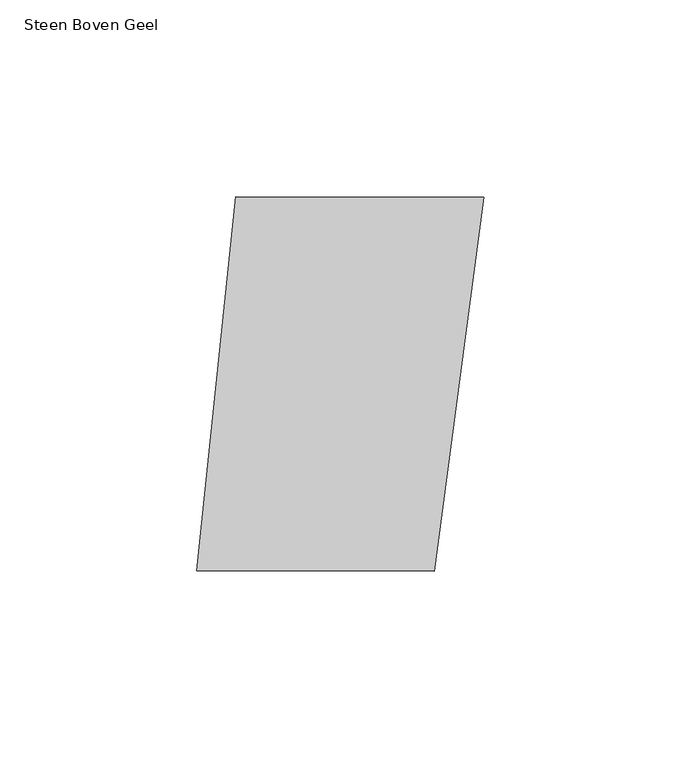
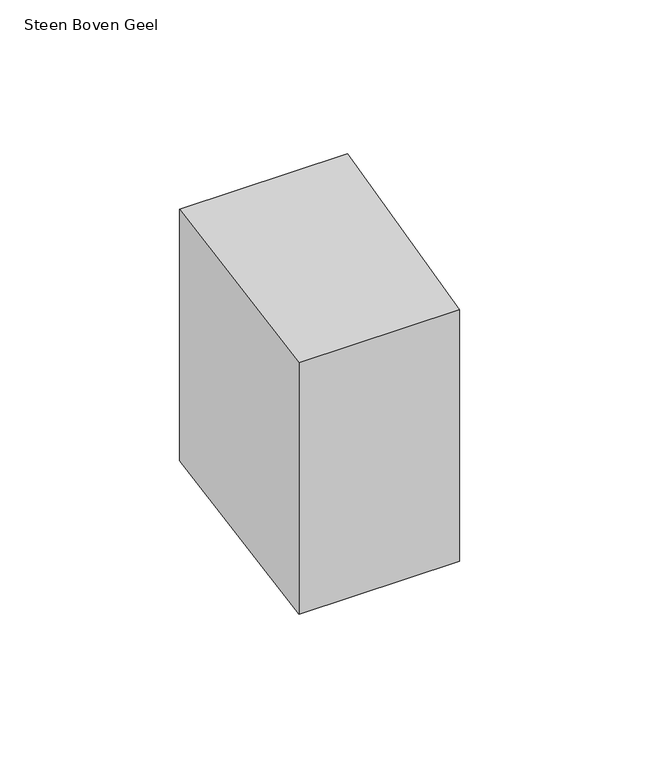
"""IFC4 building model written with IfcOpenShell, lengths in millimetres: proxy geometry, 00_GMA_steen_versie_4 : Steen Boven Geel."""

from ifc_helpers import new_model, si_unit, origin, origin_with_axes, place, context, project, spatial, polyline, outline, extrude, source, transform, mapped, element, save


def steen_boven_geel_28c625b8(model_context):
    return source(origin(), model_context, "Body", "SweptSolid", [
        extrude(outline(polyline([(107.1916785, 118.5943168), (94.5727762, 23.5682858), (34.2758002, 23.6569612), (44.1148033, 118.6720607), (107.1916785, 118.5943168)])), origin_with_axes(), (0.0, 0.0, 1.0), 100.0),
    ])


if __name__ == "__main__":
    model = new_model("IFC4")
    model_context = context("Model", 3, world=origin())
    ifc_project = project(units=[si_unit("LENGTHUNIT", "METRE", prefix="MILLI")], contexts=[model_context])
    site = spatial("IfcSite", under=ifc_project)
    building = spatial("IfcBuilding", under=site)
    placement = place(None, origin())
    steen_boven_geel_shape = steen_boven_geel_28c625b8(model_context)
    element("IfcBuildingElementProxy", 1, Name="00_GMA_steen_versie_4 : Steen Boven Geel", ObjectType="00_GMA_steen_versie_4 : Steen Boven Geel", at=placement, inside=building, context=model_context, shape_type="MappedRepresentation", body=[
        mapped(steen_boven_geel_shape, transform((0.0, 0.0, 0.0), x_axis=(1.0, 0.0, 0.0), y_axis=(0.0, 1.0, 0.0), z_axis=(0.0, 0.0, 1.0))),
    ])
    save(model, "model.ifc")

# Revit data of these elements
# Type "00_GMA_steen_versie_4 : Steen Boven Geel"
#   StootVoegHalfBoven [instance default] = 5 mm
#   StootVoegHalf [instance default] = 5 mm
#   StootVoegBreedteOnder = 10 mm
#   StootVoegBreedteBoven = 10 mm
#   Steendikte = 100 mm
#   LintVoegOnderHalf = 5 mm
#   LintVoegOnder = 10 mm
#   LintVoegBovenHalf = 0 mm
#   LintVoegBoven = 0 mm
#   materiaal = 21_steen_geel
#   MateriaalVoeg = none
#   Default Elevation = 0
# Element 1 (IfcBuildingElementProxy, "00_GMA_steen_versie_4 : Steen Boven Geel")
#   Materials on its faces: "21_steen_geel"
# Materials
#   "21_steen_geel": class "Unassigned", colour RGB 202 202 0, transparency 0, Cost = 0
